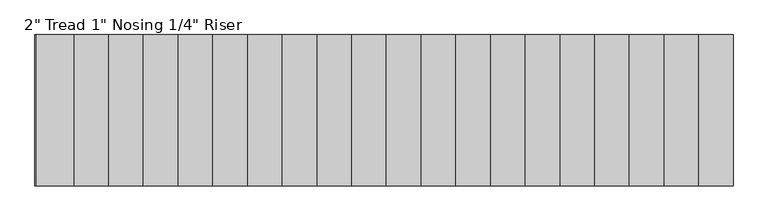
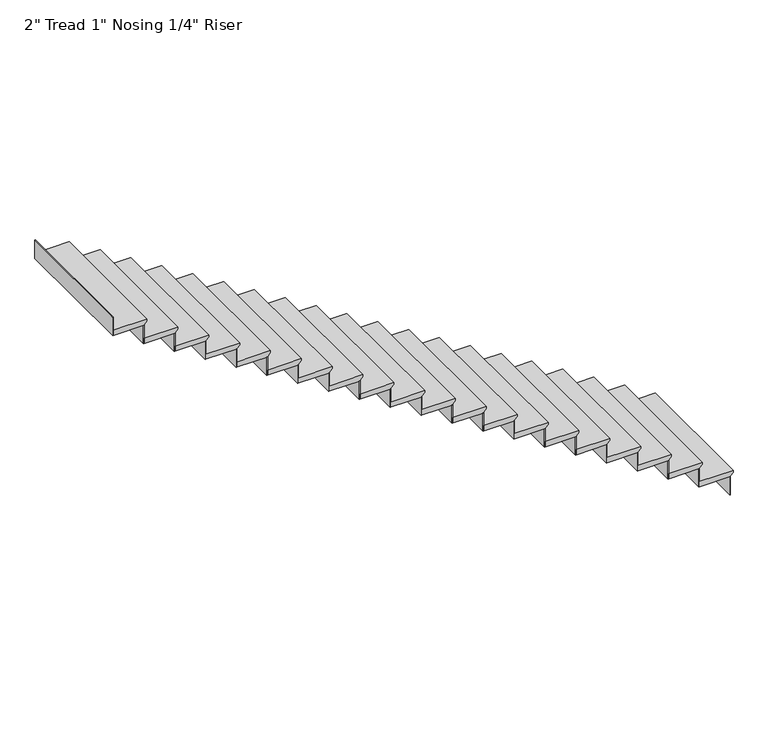
"""IFC4 building model written with IfcOpenShell, lengths in millimetres: stair flight geometry."""

from ifc_helpers import new_model, si_unit, frame, origin, place, context, project, spatial, polyline, outline, extrude, source, transform, mapped, element, save


def stair_flight_7109dd71(model_context):
    return source(origin(), model_context, "Body", "SweptSolid", [
        extrude(outline(polyline([(1393.3714286, -4798.5507921), (1393.3714286, -5103.3507921), (1342.5714286, -5103.3507921), (1342.5714286, -4823.9507921), (1348.9214286, -4823.9507921), (1374.3214286, -4798.5507921), (1393.3714286, -4798.5507921)])), frame((0.0, -4109.6601743, 0.0), z_axis=(0.0, 1.0, 0.0), x_axis=(0.0, 0.0, 1.0)), (0.0, 0.0, 1.0), 1219.2),
        extrude(outline(polyline([(-4830.3007921, -2890.4601743), (-4823.9507921, -2890.4601743), (-4823.9507921, -4109.6601743), (-4830.3007921, -4109.6601743), (-4830.3007921, -2890.4601743)])), frame((0.0, 0.0, 1168.4), z_axis=(0.0, 0.0, 1.0), x_axis=(1.0, 0.0, 0.0)), (0.0, 0.0, 1.0), 174.1714286),
        extrude(outline(polyline([(-5109.7007921, -2890.4601743), (-5103.3507921, -2890.4601743), (-5103.3507921, -4109.6601743), (-5109.7007921, -4109.6601743), (-5109.7007921, -2890.4601743)])), frame((0.0, 0.0, 1342.5714286), z_axis=(0.0, 0.0, 1.0), x_axis=(1.0, 0.0, 0.0)), (0.0, 0.0, 1.0), 174.1714286),
        extrude(outline(polyline([(1567.5428571, -5077.9507921), (1567.5428571, -5382.7507921), (1516.7428571, -5382.7507921), (1516.7428571, -5103.3507921), (1523.0928571, -5103.3507921), (1548.4928571, -5077.9507921), (1567.5428571, -5077.9507921)])), frame((0.0, -4109.6601743, 0.0), z_axis=(0.0, 1.0, 0.0), x_axis=(0.0, 0.0, 1.0)), (0.0, 0.0, 1.0), 1219.2),
        extrude(outline(polyline([(-5389.1007921, -2890.4601743), (-5382.7507921, -2890.4601743), (-5382.7507921, -4109.6601743), (-5389.1007921, -4109.6601743), (-5389.1007921, -2890.4601743)])), frame((0.0, 0.0, 1516.7428571), z_axis=(0.0, 0.0, 1.0), x_axis=(1.0, 0.0, 0.0)), (0.0, 0.0, 1.0), 174.1714286),
        extrude(outline(polyline([(1741.7142857, -5357.3507921), (1741.7142857, -5662.1507921), (1690.9142857, -5662.1507921), (1690.9142857, -5382.7507921), (1697.2642857, -5382.7507921), (1722.6642857, -5357.3507921), (1741.7142857, -5357.3507921)])), frame((0.0, -4109.6601743, 0.0), z_axis=(0.0, 1.0, 0.0), x_axis=(0.0, 0.0, 1.0)), (0.0, 0.0, 1.0), 1219.2),
        extrude(outline(polyline([(-5668.5007921, -2890.4601743), (-5662.1507921, -2890.4601743), (-5662.1507921, -4109.6601743), (-5668.5007921, -4109.6601743), (-5668.5007921, -2890.4601743)])), frame((0.0, 0.0, 1690.9142857), z_axis=(0.0, 0.0, 1.0), x_axis=(1.0, 0.0, 0.0)), (0.0, 0.0, 1.0), 174.1714286),
        extrude(outline(polyline([(1915.8857143, -5636.7507921), (1915.8857143, -5941.5507921), (1865.0857143, -5941.5507921), (1865.0857143, -5662.1507921), (1871.4357143, -5662.1507921), (1896.8357143, -5636.7507921), (1915.8857143, -5636.7507921)])), frame((0.0, -4109.6601743, 0.0), z_axis=(0.0, 1.0, 0.0), x_axis=(0.0, 0.0, 1.0)), (0.0, 0.0, 1.0), 1219.2),
        extrude(outline(polyline([(-5947.9007921, -2890.4601743), (-5941.5507921, -2890.4601743), (-5941.5507921, -4109.6601743), (-5947.9007921, -4109.6601743), (-5947.9007921, -2890.4601743)])), frame((0.0, 0.0, 1865.0857143), z_axis=(0.0, 0.0, 1.0), x_axis=(1.0, 0.0, 0.0)), (0.0, 0.0, 1.0), 174.1714286),
        extrude(outline(polyline([(2090.0571429, -5916.1507921), (2090.0571429, -6220.9507921), (2039.2571429, -6220.9507921), (2039.2571429, -5941.5507921), (2045.6071429, -5941.5507921), (2071.0071429, -5916.1507921), (2090.0571429, -5916.1507921)])), frame((0.0, -4109.6601743, 0.0), z_axis=(0.0, 1.0, 0.0), x_axis=(0.0, 0.0, 1.0)), (0.0, 0.0, 1.0), 1219.2),
        extrude(outline(polyline([(-6227.3007921, -2890.4601743), (-6220.9507921, -2890.4601743), (-6220.9507921, -4109.6601743), (-6227.3007921, -4109.6601743), (-6227.3007921, -2890.4601743)])), frame((0.0, 0.0, 2039.2571429), z_axis=(0.0, 0.0, 1.0), x_axis=(1.0, 0.0, 0.0)), (0.0, 0.0, 1.0), 174.1714286),
        extrude(outline(polyline([(2264.2285714, -6195.5507921), (2264.2285714, -6500.3507921), (2213.4285714, -6500.3507921), (2213.4285714, -6220.9507921), (2219.7785714, -6220.9507921), (2245.1785714, -6195.5507921), (2264.2285714, -6195.5507921)])), frame((0.0, -4109.6601743, 0.0), z_axis=(0.0, 1.0, 0.0), x_axis=(0.0, 0.0, 1.0)), (0.0, 0.0, 1.0), 1219.2),
        extrude(outline(polyline([(-6506.7007921, -2890.4601743), (-6500.3507921, -2890.4601743), (-6500.3507921, -4109.6601743), (-6506.7007921, -4109.6601743), (-6506.7007921, -2890.4601743)])), frame((0.0, 0.0, 2213.4285714), z_axis=(0.0, 0.0, 1.0), x_axis=(1.0, 0.0, 0.0)), (0.0, 0.0, 1.0), 174.1714286),
        extrude(outline(polyline([(2438.4, -6474.9507921), (2438.4, -6779.7507921), (2387.6, -6779.7507921), (2387.6, -6500.3507921), (2393.95, -6500.3507921), (2419.35, -6474.9507921), (2438.4, -6474.9507921)])), frame((0.0, -4109.6601743, 0.0), z_axis=(0.0, 1.0, 0.0), x_axis=(0.0, 0.0, 1.0)), (0.0, 0.0, 1.0), 1219.2),
        extrude(outline(polyline([(-6786.1007921, -2890.4601743), (-6779.7507921, -2890.4601743), (-6779.7507921, -4109.6601743), (-6786.1007921, -4109.6601743), (-6786.1007921, -2890.4601743)])), frame((0.0, 0.0, 2387.6), z_axis=(0.0, 0.0, 1.0), x_axis=(1.0, 0.0, 0.0)), (0.0, 0.0, 1.0), 174.1714286),
        extrude(outline(polyline([(2612.5714286, -6754.3507921), (2612.5714286, -7059.1507921), (2561.7714286, -7059.1507921), (2561.7714286, -6779.7507921), (2568.1214286, -6779.7507921), (2593.5214286, -6754.3507921), (2612.5714286, -6754.3507921)])), frame((0.0, -4109.6601743, 0.0), z_axis=(0.0, 1.0, 0.0), x_axis=(0.0, 0.0, 1.0)), (0.0, 0.0, 1.0), 1219.2),
        extrude(outline(polyline([(-7065.5007921, -2890.4601743), (-7059.1507921, -2890.4601743), (-7059.1507921, -4109.6601743), (-7065.5007921, -4109.6601743), (-7065.5007921, -2890.4601743)])), frame((0.0, 0.0, 2561.7714286), z_axis=(0.0, 0.0, 1.0), x_axis=(1.0, 0.0, 0.0)), (0.0, 0.0, 1.0), 174.1714286),
        extrude(outline(polyline([(2786.7428571, -7033.7507921), (2786.7428571, -7338.5507921), (2735.9428571, -7338.5507921), (2735.9428571, -7059.1507921), (2742.2928571, -7059.1507921), (2767.6928571, -7033.7507921), (2786.7428571, -7033.7507921)])), frame((0.0, -4109.6601743, 0.0), z_axis=(0.0, 1.0, 0.0), x_axis=(0.0, 0.0, 1.0)), (0.0, 0.0, 1.0), 1219.2),
        extrude(outline(polyline([(-7344.9007921, -2890.4601743), (-7338.5507921, -2890.4601743), (-7338.5507921, -4109.6601743), (-7344.9007921, -4109.6601743), (-7344.9007921, -2890.4601743)])), frame((0.0, 0.0, 2735.9428571), z_axis=(0.0, 0.0, 1.0), x_axis=(1.0, 0.0, 0.0)), (0.0, 0.0, 1.0), 174.1714286),
        extrude(outline(polyline([(2960.9142857, -7313.1507921), (2960.9142857, -7617.9507921), (2910.1142857, -7617.9507921), (2910.1142857, -7338.5507921), (2916.4642857, -7338.5507921), (2941.8642857, -7313.1507921), (2960.9142857, -7313.1507921)])), frame((0.0, -4109.6601743, 0.0), z_axis=(0.0, 1.0, 0.0), x_axis=(0.0, 0.0, 1.0)), (0.0, 0.0, 1.0), 1219.2),
        extrude(outline(polyline([(-7624.3007921, -2890.4601743), (-7617.9507921, -2890.4601743), (-7617.9507921, -4109.6601743), (-7624.3007921, -4109.6601743), (-7624.3007921, -2890.4601743)])), frame((0.0, 0.0, 2910.1142857), z_axis=(0.0, 0.0, 1.0), x_axis=(1.0, 0.0, 0.0)), (0.0, 0.0, 1.0), 174.1714286),
        extrude(outline(polyline([(3135.0857143, -7592.5507921), (3135.0857143, -7897.3507921), (3084.2857143, -7897.3507921), (3084.2857143, -7617.9507921), (3090.6357143, -7617.9507921), (3116.0357143, -7592.5507921), (3135.0857143, -7592.5507921)])), frame((0.0, -4109.6601743, 0.0), z_axis=(0.0, 1.0, 0.0), x_axis=(0.0, 0.0, 1.0)), (0.0, 0.0, 1.0), 1219.2),
        extrude(outline(polyline([(-7903.7007921, -2890.4601743), (-7897.3507921, -2890.4601743), (-7897.3507921, -4109.6601743), (-7903.7007921, -4109.6601743), (-7903.7007921, -2890.4601743)])), frame((0.0, 0.0, 3084.2857143), z_axis=(0.0, 0.0, 1.0), x_axis=(1.0, 0.0, 0.0)), (0.0, 0.0, 1.0), 174.1714286),
        extrude(outline(polyline([(3309.2571429, -7871.9507921), (3309.2571429, -8176.7507921), (3258.4571429, -8176.7507921), (3258.4571429, -7897.3507921), (3264.8071429, -7897.3507921), (3290.2071429, -7871.9507921), (3309.2571429, -7871.9507921)])), frame((0.0, -4109.6601743, 0.0), z_axis=(0.0, 1.0, 0.0), x_axis=(0.0, 0.0, 1.0)), (0.0, 0.0, 1.0), 1219.2),
        extrude(outline(polyline([(-8183.1007921, -2890.4601743), (-8176.7507921, -2890.4601743), (-8176.7507921, -4109.6601743), (-8183.1007921, -4109.6601743), (-8183.1007921, -2890.4601743)])), frame((0.0, 0.0, 3258.4571429), z_axis=(0.0, 0.0, 1.0), x_axis=(1.0, 0.0, 0.0)), (0.0, 0.0, 1.0), 174.1714286),
        extrude(outline(polyline([(3483.4285714, -8151.3507921), (3483.4285714, -8456.1507921), (3432.6285714, -8456.1507921), (3432.6285714, -8176.7507921), (3438.9785714, -8176.7507921), (3464.3785714, -8151.3507921), (3483.4285714, -8151.3507921)])), frame((0.0, -4109.6601743, 0.0), z_axis=(0.0, 1.0, 0.0), x_axis=(0.0, 0.0, 1.0)), (0.0, 0.0, 1.0), 1219.2),
        extrude(outline(polyline([(-8462.5007921, -2890.4601743), (-8456.1507921, -2890.4601743), (-8456.1507921, -4109.6601743), (-8462.5007921, -4109.6601743), (-8462.5007921, -2890.4601743)])), frame((0.0, 0.0, 3432.6285714), z_axis=(0.0, 0.0, 1.0), x_axis=(1.0, 0.0, 0.0)), (0.0, 0.0, 1.0), 174.1714286),
        extrude(outline(polyline([(3657.6, -8430.7507921), (3657.6, -8735.5507921), (3606.8, -8735.5507921), (3606.8, -8456.1507921), (3613.15, -8456.1507921), (3638.55, -8430.7507921), (3657.6, -8430.7507921)])), frame((0.0, -4109.6601743, 0.0), z_axis=(0.0, 1.0, 0.0), x_axis=(0.0, 0.0, 1.0)), (0.0, 0.0, 1.0), 1219.2),
        extrude(outline(polyline([(-8741.9007921, -2890.4601743), (-8735.5507921, -2890.4601743), (-8735.5507921, -4109.6601743), (-8741.9007921, -4109.6601743), (-8741.9007921, -2890.4601743)])), frame((0.0, 0.0, 3606.8), z_axis=(0.0, 0.0, 1.0), x_axis=(1.0, 0.0, 0.0)), (0.0, 0.0, 1.0), 174.1714286),
        extrude(outline(polyline([(3831.7714286, -8710.1507921), (3831.7714286, -9014.9507921), (3780.9714286, -9014.9507921), (3780.9714286, -8735.5507921), (3787.3214286, -8735.5507921), (3812.7214286, -8710.1507921), (3831.7714286, -8710.1507921)])), frame((0.0, -4109.6601743, 0.0), z_axis=(0.0, 1.0, 0.0), x_axis=(0.0, 0.0, 1.0)), (0.0, 0.0, 1.0), 1219.2),
        extrude(outline(polyline([(-9021.3007921, -2890.4601743), (-9014.9507921, -2890.4601743), (-9014.9507921, -4109.6601743), (-9021.3007921, -4109.6601743), (-9021.3007921, -2890.4601743)])), frame((0.0, 0.0, 3780.9714286), z_axis=(0.0, 0.0, 1.0), x_axis=(1.0, 0.0, 0.0)), (0.0, 0.0, 1.0), 174.1714286),
        extrude(outline(polyline([(4005.9428571, -8989.5507921), (4005.9428571, -9294.3507921), (3955.1428571, -9294.3507921), (3955.1428571, -9014.9507921), (3961.4928571, -9014.9507921), (3986.8928571, -8989.5507921), (4005.9428571, -8989.5507921)])), frame((0.0, -4109.6601743, 0.0), z_axis=(0.0, 1.0, 0.0), x_axis=(0.0, 0.0, 1.0)), (0.0, 0.0, 1.0), 1219.2),
        extrude(outline(polyline([(-9300.7007921, -2890.4601743), (-9294.3507921, -2890.4601743), (-9294.3507921, -4109.6601743), (-9300.7007921, -4109.6601743), (-9300.7007921, -2890.4601743)])), frame((0.0, 0.0, 3955.1428571), z_axis=(0.0, 0.0, 1.0), x_axis=(1.0, 0.0, 0.0)), (0.0, 0.0, 1.0), 174.1714286),
        extrude(outline(polyline([(4180.1142857, -9268.9507921), (4180.1142857, -9573.7507921), (4129.3142857, -9573.7507921), (4129.3142857, -9294.3507921), (4135.6642857, -9294.3507921), (4161.0642857, -9268.9507921), (4180.1142857, -9268.9507921)])), frame((0.0, -4109.6601743, 0.0), z_axis=(0.0, 1.0, 0.0), x_axis=(0.0, 0.0, 1.0)), (0.0, 0.0, 1.0), 1219.2),
        extrude(outline(polyline([(-9580.1007921, -2890.4601743), (-9573.7507921, -2890.4601743), (-9573.7507921, -4109.6601743), (-9580.1007921, -4109.6601743), (-9580.1007921, -2890.4601743)])), frame((0.0, 0.0, 4129.3142857), z_axis=(0.0, 0.0, 1.0), x_axis=(1.0, 0.0, 0.0)), (0.0, 0.0, 1.0), 174.1714286),
        extrude(outline(polyline([(4354.2857143, -9548.3507921), (4354.2857143, -9853.1507921), (4303.4857143, -9853.1507921), (4303.4857143, -9573.7507921), (4309.8357143, -9573.7507921), (4335.2357143, -9548.3507921), (4354.2857143, -9548.3507921)])), frame((0.0, -4109.6601743, 0.0), z_axis=(0.0, 1.0, 0.0), x_axis=(0.0, 0.0, 1.0)), (0.0, 0.0, 1.0), 1219.2),
        extrude(outline(polyline([(-9859.5007921, -2890.4601743), (-9853.1507921, -2890.4601743), (-9853.1507921, -4109.6601743), (-9859.5007921, -4109.6601743), (-9859.5007921, -2890.4601743)])), frame((0.0, 0.0, 4303.4857143), z_axis=(0.0, 0.0, 1.0), x_axis=(1.0, 0.0, 0.0)), (0.0, 0.0, 1.0), 174.1714286),
        extrude(outline(polyline([(4528.4571429, -9827.7507921), (4528.4571429, -10132.5507921), (4477.6571429, -10132.5507921), (4477.6571429, -9853.1507921), (4484.0071429, -9853.1507921), (4509.4071429, -9827.7507921), (4528.4571429, -9827.7507921)])), frame((0.0, -4109.6601743, 0.0), z_axis=(0.0, 1.0, 0.0), x_axis=(0.0, 0.0, 1.0)), (0.0, 0.0, 1.0), 1219.2),
        extrude(outline(polyline([(-10138.9007921, -2890.4601743), (-10132.5507921, -2890.4601743), (-10132.5507921, -4109.6601743), (-10138.9007921, -4109.6601743), (-10138.9007921, -2890.4601743)])), frame((0.0, 0.0, 4477.6571429), z_axis=(0.0, 0.0, 1.0), x_axis=(1.0, 0.0, 0.0)), (0.0, 0.0, 1.0), 174.1714286),
        extrude(outline(polyline([(-10418.3007921, -2890.4601743), (-10411.9507921, -2890.4601743), (-10411.9507921, -4109.6601743), (-10418.3007921, -4109.6601743), (-10418.3007921, -2890.4601743)])), frame((0.0, 0.0, 4651.8285714), z_axis=(0.0, 0.0, 1.0), x_axis=(1.0, 0.0, 0.0)), (0.0, 0.0, 1.0), 174.1714286),
        extrude(outline(polyline([(4702.6285714, -10107.1507921), (4702.6285714, -10411.9507921), (4651.8285714, -10411.9507921), (4651.8285714, -10132.5507921), (4658.1785714, -10132.5507921), (4683.5785714, -10107.1507921), (4702.6285714, -10107.1507921)])), frame((0.0, -4109.6601743, 0.0), z_axis=(0.0, 1.0, 0.0), x_axis=(0.0, 0.0, 1.0)), (0.0, 0.0, 1.0), 1219.2),
    ])


if __name__ == "__main__":
    model = new_model("IFC4")
    model_context = context("Model", 3, world=origin())
    ifc_project = project(units=[si_unit("LENGTHUNIT", "METRE", prefix="MILLI")], contexts=[model_context])
    site = spatial("IfcSite", under=ifc_project)
    building = spatial("IfcBuilding", under=site)
    placement = place(None, origin())
    stair_flight_shape = stair_flight_7109dd71(model_context)
    element("IfcStairFlight", 1, ObjectType="2\" Tread 1\" Nosing 1/4\" Riser", at=placement, inside=building, context=model_context, shape_type="MappedRepresentation", body=[
        mapped(stair_flight_shape, transform((0.0, 0.0, 0.0), x_axis=(1.0, 0.0, 0.0), y_axis=(0.0, 1.0, 0.0), z_axis=(0.0, 0.0, 1.0))),
    ])
    save(model, "model.ifc")
